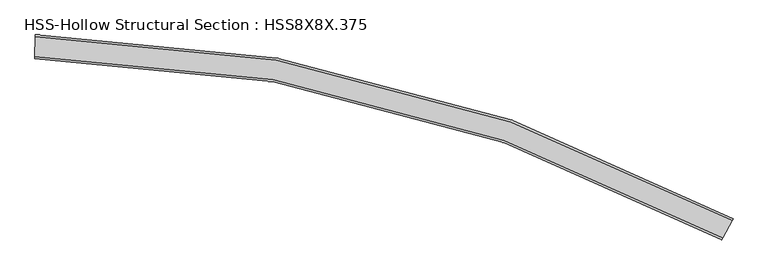
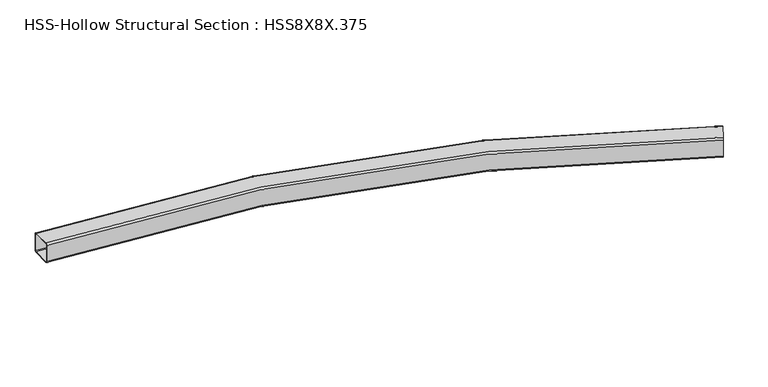
"""IFC4 building model written with IfcOpenShell, lengths in millimetres: beam geometry, HSS-Hollow Structural Section : HSS8X8X.375."""

from ifc_helpers import new_model, si_unit, point, frame, origin, place, context, project, spatial, polyline, circle_curve, ellipse_curve, trimmed, source, transform, mapped, element, save
from ifc_brep_helpers import plane_surface, cylinder_surface, revolved_surface, advanced_brep


def hss_hollow_structural_section_hss8x8x_375_3f7a212a(model_context):
    return source(origin(), model_context, "Body", "AdvancedBrep", [
        advanced_brep(
        [(6121.7238156, -1466.3923014, 83.9390625), (6113.2336242, -1481.8785974, 101.6), (6032.5291082, -1629.0854109, 101.6), (6024.0389168, -1644.5717069, 83.9390625), (6024.0389168, -1644.5717069, -83.9390625), (6032.5291082, -1629.0854109, -101.6), (6113.2336242, -1481.8785974, -101.6), (6121.7238156, -1466.3923014, -83.9390625), (6032.5291082, -1629.0854109, 92.7695312), (6113.2336242, -1481.8785974, 92.7695312), (6117.4787199, -1474.1354494, 83.9390625), (6117.4787199, -1474.1354494, -83.9390625), (6113.2336242, -1481.8785974, -92.7695313), (6032.5291082, -1629.0854109, -92.7695313), (6028.2840125, -1636.8285589, -83.9390625), (6028.2840125, -1636.8285589, 83.9390625), (187.7413355, 100.2159767, 83.9390625), (187.7413355, 100.2159767, -83.9390625), (187.4809579, 82.5569587, -101.6), (185.0059077, -85.3029203, -101.6), (184.7455301, -102.9619383, -83.9390625), (184.7455301, -102.9619383, 83.9390625), (185.0059077, -85.3029203, 101.6), (187.4809579, 82.5569587, 101.6), (185.0059077, -85.3029203, 92.7695312), (184.8757189, -94.1324293, 83.9390625), (184.8757189, -94.1324293, -83.9390625), (185.0059077, -85.3029203, -92.7695313), (187.4809579, 82.5569587, -92.7695313), (187.6111467, 91.3864677, -83.9390625), (187.6111467, 91.3864677, 83.9390625), (187.4809579, 82.5569587, 92.7695312)],
        [
            (0, 1, circle_curve(frame((6113.2336242, -1481.8785974, 83.9390625), z_axis=(0.8768671529491877, -0.4807327699239839, 0.0), x_axis=(-0.4807327699239839, -0.8768671529491877, 0.0)), 17.6609375)),
            (1, 2),
            (2, 3, circle_curve(frame((6032.5291082, -1629.0854109, 83.9390625), z_axis=(0.8768671529491877, -0.4807327699239839, 0.0), x_axis=(-0.4807327699239839, -0.8768671529491877, 0.0)), 17.6609375)),
            (3, 4),
            (4, 5, circle_curve(frame((6032.5291082, -1629.0854109, -83.9390625), z_axis=(0.8768671529491877, -0.4807327699239839, 0.0), x_axis=(-0.4807327699239839, -0.8768671529491877, 0.0)), 17.6609375)),
            (5, 6),
            (6, 7, circle_curve(frame((6113.2336242, -1481.8785974, -83.9390625), z_axis=(0.8768671529491877, -0.4807327699239839, 0.0), x_axis=(-0.4807327699239839, -0.8768671529491877, 0.0)), 17.6609375)),
            (7, 0),
            (8, 9),
            (9, 10, circle_curve(frame((6113.2336242, -1481.8785974, 83.9390625), z_axis=(-0.8768671529491877, 0.4807327699239839, 0.0), x_axis=(-0.4807327699239839, -0.8768671529491877, 0.0)), 8.8304688)),
            (10, 11),
            (11, 12, circle_curve(frame((6113.2336242, -1481.8785974, -83.9390625), z_axis=(-0.8768671529491877, 0.4807327699239839, 0.0), x_axis=(-0.4807327699239839, -0.8768671529491877, 0.0)), 8.8304688)),
            (12, 13),
            (13, 14, circle_curve(frame((6032.5291082, -1629.0854109, -83.9390625), z_axis=(-0.8768671529491877, 0.4807327699239839, 0.0), x_axis=(-0.4807327699239839, -0.8768671529491877, 0.0)), 8.8304688)),
            (14, 15),
            (15, 8, circle_curve(frame((6032.5291082, -1629.0854109, 83.9390625), z_axis=(-0.8768671529491877, 0.4807327699239839, 0.0), x_axis=(-0.4807327699239839, -0.8768671529491877, 0.0)), 8.8304688)),
            (16, 17),
            (17, 18, circle_curve(frame((187.4809579, 82.5569587, -83.9390625), z_axis=(-0.999891314050926, 0.014743136895265851, 0.0), x_axis=(-0.014743136895265851, -0.999891314050926, 0.0)), 17.6609375)),
            (18, 19),
            (19, 20, circle_curve(frame((185.0059077, -85.3029203, -83.9390625), z_axis=(-0.999891314050926, 0.014743136895265851, 0.0), x_axis=(-0.014743136895265851, -0.999891314050926, 0.0)), 17.6609375)),
            (20, 21),
            (21, 22, circle_curve(frame((185.0059077, -85.3029203, 83.9390625), z_axis=(-0.999891314050926, 0.014743136895265851, 0.0), x_axis=(-0.014743136895265851, -0.999891314050926, 0.0)), 17.6609375)),
            (22, 23),
            (23, 16, circle_curve(frame((187.4809579, 82.5569587, 83.9390625), z_axis=(-0.999891314050926, 0.014743136895265851, 0.0), x_axis=(-0.014743136895265851, -0.999891314050926, 0.0)), 17.6609375)),
            (24, 25, circle_curve(frame((185.0059077, -85.3029203, 83.9390625), z_axis=(0.999891314050926, -0.014743136895265851, 0.0), x_axis=(-0.014743136895265851, -0.999891314050926, 0.0)), 8.8304688)),
            (25, 26),
            (26, 27, circle_curve(frame((185.0059077, -85.3029203, -83.9390625), z_axis=(0.999891314050926, -0.014743136895265851, 0.0), x_axis=(-0.014743136895265851, -0.999891314050926, 0.0)), 8.8304688)),
            (27, 28),
            (28, 29, circle_curve(frame((187.4809579, 82.5569587, -83.9390625), z_axis=(0.999891314050926, -0.014743136895265851, 0.0), x_axis=(-0.014743136895265851, -0.999891314050926, 0.0)), 8.8304688)),
            (29, 30),
            (30, 31, circle_curve(frame((187.4809579, 82.5569587, 83.9390625), z_axis=(0.999891314050926, -0.014743136895265851, 0.0), x_axis=(-0.014743136895265851, -0.999891314050926, 0.0)), 8.8304688)),
            (31, 24),
            (0, 16, circle_curve(frame((0.0, -12632.5512762, 83.9390625), z_axis=(0.0, 0.0, 1.0), x_axis=(-0.5014171979932397, -0.8652056365723748, 0.0)), 12734.1512762)),
            (23, 1, circle_curve(frame((0.0, -12632.5512762, 101.6), z_axis=(0.0, 0.0, -1.0), x_axis=(-0.5014171979932397, -0.8652056365723748, 0.0)), 12716.4903387)),
            (22, 2, circle_curve(frame((0.0, -12632.5512762, 101.6), z_axis=(0.0, 0.0, -1.0), x_axis=(-0.5014171979932397, -0.8652056365723748, 0.0)), 12548.6122137)),
            (21, 3, circle_curve(frame((0.0, -12632.5512762, 83.9390625), z_axis=(0.0, 0.0, -1.0), x_axis=(-0.5014171979932397, -0.8652056365723748, 0.0)), 12530.9512762)),
            (20, 4, circle_curve(frame((0.0, -12632.5512762, -83.9390625), z_axis=(0.0, 0.0, -1.0), x_axis=(-0.5014171979932397, -0.8652056365723748, 0.0)), 12530.9512762)),
            (19, 5, circle_curve(frame((0.0, -12632.5512762, -101.6), z_axis=(0.0, 0.0, -1.0), x_axis=(-0.5014171979932397, -0.8652056365723748, 0.0)), 12548.6122137)),
            (18, 6, circle_curve(frame((0.0, -12632.5512762, -101.6), z_axis=(0.0, 0.0, -1.0), x_axis=(-0.5014171979932397, -0.8652056365723748, 0.0)), 12716.4903387)),
            (17, 7, circle_curve(frame((0.0, -12632.5512762, -83.9390625), z_axis=(0.0, 0.0, -1.0), x_axis=(-0.5014171979932397, -0.8652056365723748, 0.0)), 12734.1512762)),
            (8, 24, circle_curve(frame((0.0, -12632.5512762, 92.7695312), z_axis=(0.0, 0.0, 1.0), x_axis=(-0.5014171979932397, -0.8652056365723748, 0.0)), 12548.6122137)),
            (31, 9, circle_curve(frame((0.0, -12632.5512762, 92.7695312), z_axis=(0.0, 0.0, -1.0), x_axis=(-0.5014171979932397, -0.8652056365723748, 0.0)), 12716.4903387)),
            (30, 10, circle_curve(frame((0.0, -12632.5512762, 83.9390625), z_axis=(0.0, 0.0, -1.0), x_axis=(-0.5014171979932397, -0.8652056365723748, 0.0)), 12725.3208075)),
            (29, 11, circle_curve(frame((0.0, -12632.5512762, -83.9390625), z_axis=(0.0, 0.0, -1.0), x_axis=(-0.5014171979932397, -0.8652056365723748, 0.0)), 12725.3208075)),
            (28, 12, circle_curve(frame((0.0, -12632.5512762, -92.7695313), z_axis=(0.0, 0.0, -1.0), x_axis=(-0.5014171979932397, -0.8652056365723748, 0.0)), 12716.4903387)),
            (27, 13, circle_curve(frame((0.0, -12632.5512762, -92.7695313), z_axis=(0.0, 0.0, -1.0), x_axis=(-0.5014171979932397, -0.8652056365723748, 0.0)), 12548.6122137)),
            (26, 14, circle_curve(frame((0.0, -12632.5512762, -83.9390625), z_axis=(0.0, 0.0, -1.0), x_axis=(-0.5014171979932397, -0.8652056365723748, 0.0)), 12539.781745)),
            (25, 15, circle_curve(frame((0.0, -12632.5512762, 83.9390625), z_axis=(0.0, 0.0, -1.0), x_axis=(-0.5014171979932397, -0.8652056365723748, 0.0)), 12539.781745)),
        ],
        [
            plane_surface(frame((6072.8813662, -1555.4820042, 0.0), z_axis=(0.8768671529491846, -0.4807327699239896, 0.0), x_axis=(0.0, 0.0, 1.0))),
            plane_surface(frame((186.2434328, -1.3729808, 0.0), z_axis=(-0.9998913140509259, 0.014743136895272237, 0.0), x_axis=(0.0, 0.0, 1.0))),
            revolved_surface(trimmed(ellipse_curve(frame((-6376.2669539, -23634.9303947, 83.9390625), z_axis=(0.865205636572378, -0.5014171979932341, 0.0), x_axis=(0.5014171979932341, 0.865205636572378, 0.0)), 17.6609375, 17.6609375), [point((-6376.2669539, -23634.9303947, 101.6))], [point((-6385.1224517, -23650.2107374, 83.9390625))], True, "CARTESIAN"), (0.0, -12632.5512762, 0.0), (0.0, 0.0, -1.0)),
            plane_surface(frame((0.0, -12632.5512762, 101.6), z_axis=(0.0, 0.0, 1.0), x_axis=(-0.5014171979932397, -0.8652056365723748, 0.0))),
            revolved_surface(trimmed(ellipse_curve(frame((-6292.0899749, -23489.6812947, 83.9390625), z_axis=(0.865205636572378, -0.5014171979932341, 0.0), x_axis=(0.5014171979932341, 0.865205636572378, 0.0)), 17.6609375, 17.6609375), [point((-6283.2344771, -23474.400952, 83.9390625))], [point((-6292.0899749, -23489.6812947, 101.6))], True, "CARTESIAN"), (0.0, -12632.5512762, 0.0), (0.0, 0.0, -1.0)),
            revolved_surface(polyline([(-6283.234477102014, -23474.400951982032, -83.9390625), (-6283.234477102014, -23474.400951982032, 83.9390625)]), (0.0, -12632.5512762, 0.0), (0.0, 0.0, -1.0)),
            revolved_surface(trimmed(ellipse_curve(frame((-6292.0899749, -23489.6812947, -83.9390625), z_axis=(0.865205636572378, -0.5014171979932341, 0.0), x_axis=(0.5014171979932341, 0.865205636572378, 0.0)), 17.6609375, 17.6609375), [point((-6292.0899749, -23489.6812947, -101.6))], [point((-6283.2344771, -23474.400952, -83.9390625))], True, "CARTESIAN"), (0.0, -12632.5512762, 0.0), (0.0, 0.0, -1.0)),
            plane_surface(frame((0.0, -12632.5512762, -101.6), z_axis=(0.0, 0.0, -1.0), x_axis=(-0.5014171979932397, -0.8652056365723748, 0.0))),
            revolved_surface(trimmed(ellipse_curve(frame((-6376.2669539, -23634.9303947, -83.9390625), z_axis=(0.865205636572378, -0.5014171979932341, 0.0), x_axis=(0.5014171979932341, 0.865205636572378, 0.0)), 17.6609375, 17.6609375), [point((-6385.1224517, -23650.2107374, -83.9390625))], [point((-6376.2669539, -23634.9303947, -101.6))], True, "CARTESIAN"), (0.0, -12632.5512762, 0.0), (0.0, 0.0, -1.0)),
            cylinder_surface(frame((0.0, -12632.5512762, 0.0), z_axis=(0.0, 0.0, -1.0), x_axis=(-0.5014171979932397, -0.8652056365723748, 0.0)), 12734.1512762),
            plane_surface(frame((0.0, -12632.5512762, 92.7695312), z_axis=(0.0, 0.0, -1.0), x_axis=(-0.5014171979932397, -0.8652056365723748, 0.0))),
            revolved_surface(trimmed(ellipse_curve(frame((-6376.2669539, -23634.9303947, 83.9390625), z_axis=(-0.865205636572378, 0.5014171979932341, 0.0), x_axis=(0.5014171979932341, 0.865205636572378, 0.0)), 8.8304688, 8.8304688), [point((-6380.6947028, -23642.570566, 83.9390625))], [point((-6376.2669539, -23634.9303947, 92.7695312))], True, "CARTESIAN"), (0.0, -12632.5512762, 0.0), (0.0, 0.0, -1.0)),
            revolved_surface(polyline([(-6380.6947028617205, -23642.570566040726, -83.9390625), (-6380.6947028617205, -23642.570566040726, 83.9390625)]), (0.0, -12632.5512762, 0.0), (0.0, 0.0, -1.0)),
            revolved_surface(trimmed(ellipse_curve(frame((-6376.2669539, -23634.9303947, -83.9390625), z_axis=(-0.865205636572378, 0.5014171979932341, 0.0), x_axis=(0.5014171979932341, 0.865205636572378, 0.0)), 8.8304688, 8.8304688), [point((-6376.2669539, -23634.9303947, -92.7695313))], [point((-6380.6947028, -23642.570566, -83.9390625))], True, "CARTESIAN"), (0.0, -12632.5512762, 0.0), (0.0, 0.0, -1.0)),
            plane_surface(frame((0.0, -12632.5512762, -92.7695313), z_axis=(0.0, 0.0, 1.0), x_axis=(-0.5014171979932397, -0.8652056365723748, 0.0))),
            revolved_surface(trimmed(ellipse_curve(frame((-6292.0899749, -23489.6812947, -83.9390625), z_axis=(-0.865205636572378, 0.5014171979932341, 0.0), x_axis=(0.5014171979932341, 0.865205636572378, 0.0)), 8.8304688, 8.8304688), [point((-6287.662226, -23482.0411234, -83.9390625))], [point((-6292.0899749, -23489.6812947, -92.7695313))], True, "CARTESIAN"), (0.0, -12632.5512762, 0.0), (0.0, 0.0, -1.0)),
            cylinder_surface(frame((0.0, -12632.5512762, 0.0), z_axis=(0.0, 0.0, -1.0), x_axis=(-0.5014171979932397, -0.8652056365723748, 0.0)), 12539.781745),
            revolved_surface(trimmed(ellipse_curve(frame((-6292.0899749, -23489.6812947, 83.9390625), z_axis=(-0.865205636572378, 0.5014171979932341, 0.0), x_axis=(0.5014171979932341, 0.865205636572378, 0.0)), 8.8304688, 8.8304688), [point((-6292.0899749, -23489.6812947, 92.7695312))], [point((-6287.662226, -23482.0411234, 83.9390625))], True, "CARTESIAN"), (0.0, -12632.5512762, 0.0), (0.0, 0.0, -1.0)),
        ],
        [
            (0, [[1, 2, 3, 4, 5, 6, 7, 8], [9, 10, 11, 12, 13, 14, 15, 16]]),
            (1, [[17, 18, 19, 20, 21, 22, 23, 24], [25, 26, 27, 28, 29, 30, 31, 32]]),
            (2, [[-1, 33, -24, 34]]),
            (3, [[-2, -34, -23, 35]]),
            (4, [[-3, -35, -22, 36]]),
            (5, [[-4, -36, -21, 37]]),
            (6, [[-5, -37, -20, 38]]),
            (7, [[-6, -38, -19, 39]]),
            (8, [[-7, -39, -18, 40]]),
            (9, [[-8, -40, -17, -33]]),
            (10, [[-9, 41, -32, 42]]),
            (11, [[-10, -42, -31, 43]]),
            (12, [[-11, -43, -30, 44]]),
            (13, [[-12, -44, -29, 45]]),
            (14, [[-13, -45, -28, 46]]),
            (15, [[-14, -46, -27, 47]]),
            (16, [[-15, -47, -26, 48]]),
            (17, [[-16, -48, -25, -41]]),
        ],
    ),
    ])


if __name__ == "__main__":
    model = new_model("IFC4")
    model_context = context("Model", 3, world=origin())
    ifc_project = project(units=[si_unit("LENGTHUNIT", "METRE", prefix="MILLI")], contexts=[model_context])
    site = spatial("IfcSite", under=ifc_project)
    building = spatial("IfcBuilding", under=site)
    placement = place(None, origin())
    hss_hollow_structural_section_hss8x8x_375_shape = hss_hollow_structural_section_hss8x8x_375_3f7a212a(model_context)
    element("IfcBeam", 1, ObjectType="HSS-Hollow Structural Section : HSS8X8X.375", at=placement, inside=building, context=model_context, shape_type="MappedRepresentation", body=[
        mapped(hss_hollow_structural_section_hss8x8x_375_shape, transform((0.0, 0.0, 0.0), x_axis=(1.0, 0.0, 0.0), y_axis=(0.0, 1.0, 0.0), z_axis=(0.0, 0.0, 1.0))),
    ])
    save(model, "model.ifc")

# Revit data of these elements
# Type "HSS-Hollow Structural Section : HSS8X8X.375"
#   Assembly Code = "B10"
#   Shape = "Square"
#   W = 37.6
#   Start Extension Calculation [instance default] = 10' - 0"
#   Start Extension [instance default] = -0' - 0 1/2"
#   End Extension Calculation [instance default] = 10' - 0"
#   End Extension [instance default] = -0' - 0 1/2"
#   Ht = 0' - 8"
#   Length [instance default] = 5' - 0"
#   b = 0' - 8"
#   kr = 0' - 0 89/128"
#   t = 0' - 0 89/256"
#   A = 0.0722222 SF
#   Beam Material [instance default] = Metal - Steel - ASTM A500 - Grade B - Rectangular and Square
# Element 1 (IfcBeam, "HSS-Hollow Structural Section : HSS8X8X.375")
#   Materials on its faces: "Metal - Steel - ASTM A500 - Grade B - Rectangular and Square"
# Materials
#   "Metal - Steel - ASTM A500 - Grade B - Rectangular and Square": class "Metal", colour RGB 128 0 0, transparency 0
